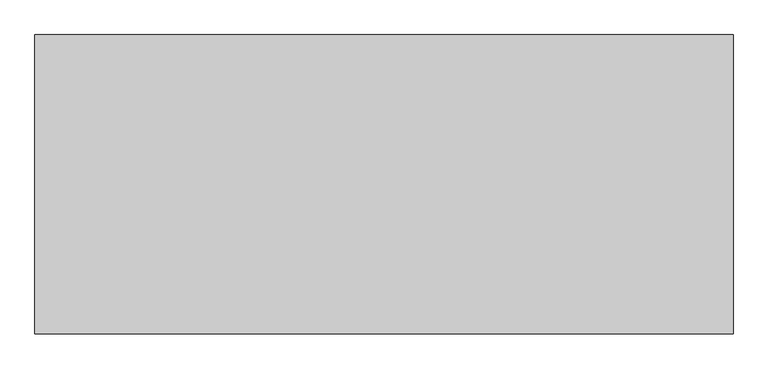
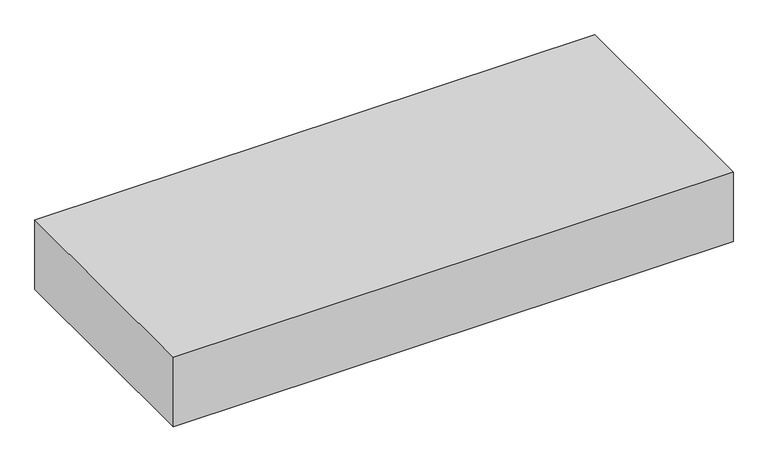
"""IFC4 building model written with IfcOpenShell, lengths in millimetres: proxy geometry, Space Planning Box_hec : Space Planning Box_hec."""

import ifcopenshell
import ifcopenshell.guid

model = None  # the IFC model being written
_history = None  # IfcOwnerHistory: only IFC2X3 demands one
_inside = {}  # id of a spatial element -> (the spatial element, [elements in it])
_under = {}  # id of a project, library or spatial element -> (it, [spatial elements below it])
_declared = {}  # id of a project -> (the project, [libraries it declares])
_typed = {}  # id of a type object -> (the type object, [elements of that type])
_made_of = {}  # id of a material, layer set ... -> (it, [elements and type objects made of it])


def new_model(schema):
    """Start an empty IFC model of exactly this schema.

    Asked for "IFC4X3", IfcOpenShell would pick the latest addendum, in which some entities
    have other attributes; the version numbers below select the first issue.
    IFC2X3 requires an IfcOwnerHistory on every rooted entity: one is made here for all.
    """
    global model, _history
    if schema == "IFC4X3":
        model = ifcopenshell.file(schema_version=(4, 3, 0, 0))
    else:
        model = ifcopenshell.file(schema=schema)
    _inside.clear()
    _under.clear()
    _declared.clear()
    _typed.clear()
    _made_of.clear()
    _history = None
    if model.schema == "IFC2X3":
        org = make("IfcOrganization", Name="unknown")
        user = make(
            "IfcPersonAndOrganization",
            ThePerson=make("IfcPerson", FamilyName="unknown"),
            TheOrganization=org,
        )
        app = make(
            "IfcApplication",
            ApplicationDeveloper=org,
            Version="unknown",
            ApplicationFullName="unknown",
            ApplicationIdentifier="unknown",
        )
        _history = make(
            "IfcOwnerHistory",
            OwningUser=user,
            OwningApplication=app,
            ChangeAction="ADDED",
            CreationDate=0,
        )
    return model


def make(cls, **values):
    """One entity of the class cls with the attributes given. An attribute that is None is left unset."""
    return model.create_entity(
        cls, **{name: value for name, value in values.items() if value is not None}
    )


def rooted(cls, **values):
    """An entity with a GlobalId (a new one), such as an element, a storey or a relation."""
    return make(cls, GlobalId=ifcopenshell.guid.new(), OwnerHistory=_history, **values)


def si_unit(unit_type, name, prefix=None):
    """IfcSIUnit, for example si_unit("LENGTHUNIT", "METRE", prefix="MILLI")."""
    return make("IfcSIUnit", UnitType=unit_type, Prefix=prefix, Name=name)


def assignment(units):
    """IfcUnitAssignment: the units of a project."""
    return None if units is None else make("IfcUnitAssignment", Units=units)


def point(xyz):
    """IfcCartesianPoint."""
    return None if xyz is None else make("IfcCartesianPoint", Coordinates=xyz)


def direction(xyz):
    """IfcDirection."""
    return None if xyz is None else make("IfcDirection", DirectionRatios=xyz)


def frame(location, z_axis=None, x_axis=None):
    """IfcAxis2Placement3D, a coordinate frame: its origin and axes. An axis left out is left unset."""
    return make(
        "IfcAxis2Placement3D",
        Location=point(location),
        Axis=direction(z_axis),
        RefDirection=direction(x_axis),
    )


def origin():
    """The frame at (0, 0, 0) with its axes left unset."""
    return frame((0.0, 0.0, 0.0))


def origin_with_axes():
    """The frame at (0, 0, 0) with the z axis (0, 0, 1) and the x axis (1, 0, 0) written out."""
    return frame((0.0, 0.0, 0.0), z_axis=(0.0, 0.0, 1.0), x_axis=(1.0, 0.0, 0.0))


def place(relative_to, where):
    """IfcLocalPlacement: puts the frame where relative to a parent placement (None: the world)."""
    return make(
        "IfcLocalPlacement", PlacementRelTo=relative_to, RelativePlacement=where
    )


def context(
    kind, dimensions, precision=None, world=None, true_north=None, identifier=None
):
    """IfcGeometricRepresentationContext, for example the 3D "Model" context."""
    return make(
        "IfcGeometricRepresentationContext",
        ContextIdentifier=identifier,
        ContextType=kind,
        CoordinateSpaceDimension=dimensions,
        Precision=precision,
        WorldCoordinateSystem=world,
        TrueNorth=true_north,
    )


def project(units=None, contexts=None):
    """IfcProject with its units and contexts."""
    return rooted(
        "IfcProject",
        Name="project",
        RepresentationContexts=contexts,
        UnitsInContext=assignment(units),
    )


def spatial(cls, under=None, at=None, **own):
    """A site, building, storey or space (cls), placed at a placement, below another one or the project."""
    s = rooted(cls, ObjectPlacement=at, **own)
    if under is not None:
        _under.setdefault(under.id(), (under, []))[1].append(s)
    return s


def polyline(points):
    """IfcPolyline through the points."""
    return make("IfcPolyline", Points=[point(p) for p in points])


def outline(outer, holes=None, kind="AREA"):
    """IfcArbitraryClosedProfileDef: a profile drawn as a closed curve; with holes, ...WithVoids."""
    if holes is None:
        return make("IfcArbitraryClosedProfileDef", ProfileType=kind, OuterCurve=outer)
    return make(
        "IfcArbitraryProfileDefWithVoids",
        ProfileType=kind,
        OuterCurve=outer,
        InnerCurves=holes,
    )


def extrude(swept, where, along, depth):
    """IfcExtrudedAreaSolid: the profile swept, set in the frame where, extruded along a direction by depth."""
    return make(
        "IfcExtrudedAreaSolid",
        SweptArea=swept,
        Position=where,
        ExtrudedDirection=direction(along),
        Depth=depth,
    )


def shape(context_of_items, identifier, shape_type, items):
    """IfcShapeRepresentation: the items that make up one representation, for example the "Body"."""
    return make(
        "IfcShapeRepresentation",
        ContextOfItems=context_of_items,
        RepresentationIdentifier=identifier,
        RepresentationType=shape_type,
        Items=items,
    )


def source(mapping_origin, context_of_items, identifier, shape_type, items):
    """IfcRepresentationMap: a shape defined once, which mapped items show again and again."""
    return make(
        "IfcRepresentationMap",
        MappingOrigin=mapping_origin,
        MappedRepresentation=shape(context_of_items, identifier, shape_type, items),
    )


def transform(
    local_origin,
    x_axis=None,
    y_axis=None,
    z_axis=None,
    scale=None,
    scale2=None,
    scale3=None,
    uniform=True,
):
    """IfcCartesianTransformationOperator3D, or its non-uniform kind. x_axis, y_axis, z_axis: its Axis1, 2, 3."""
    if uniform:
        return make(
            "IfcCartesianTransformationOperator3D",
            Axis1=direction(x_axis),
            Axis2=direction(y_axis),
            LocalOrigin=point(local_origin),
            Scale=scale,
            Axis3=direction(z_axis),
        )
    return make(
        "IfcCartesianTransformationOperator3DnonUniform",
        Axis1=direction(x_axis),
        Axis2=direction(y_axis),
        LocalOrigin=point(local_origin),
        Scale=scale,
        Axis3=direction(z_axis),
        Scale2=scale2,
        Scale3=scale3,
    )


def mapped(mapping_source, mapping_target):
    """IfcMappedItem: shows the shape of a source again, moved by a transform."""
    return make(
        "IfcMappedItem", MappingSource=mapping_source, MappingTarget=mapping_target
    )


def made_of(thing, what):
    """Note that an element or type object is made of a material, layer set ...; save() writes the relation."""
    if what is not None:
        _made_of.setdefault(what.id(), (what, []))[1].append(thing)
    return thing


def element(
    cls,
    number,
    at=None,
    inside=None,
    cuts=None,
    type_object=None,
    material=None,
    context=None,
    identifier="Body",
    shape_type=None,
    held_by="IfcProductDefinitionShape",
    body=None,
    shapes=None,
    **own,
):
    """One element of the class cls, such as IfcWall. Its Tag is "e" and its number.

    at: its placement. inside: the storey or other place that contains it. cuts: it is an
    opening in that element (IfcRelVoidsElement). A single representation is given by context,
    identifier, shape_type and body (its items); several are given by shapes. held_by: the class
    of the entity that holds the representations. save() writes the other relations.
    """
    e = rooted(cls, Tag="e%d" % number, ObjectPlacement=at, **own)
    if body is not None:
        shapes = [shape(context, identifier, shape_type, body)]
    if shapes is not None:
        e.Representation = make(held_by, Representations=shapes)
    if inside is not None:
        _inside.setdefault(inside.id(), (inside, []))[1].append(e)
    if cuts is not None:
        rooted(
            "IfcRelVoidsElement", RelatingBuildingElement=cuts, RelatedOpeningElement=e
        )
    if type_object is not None:
        _typed.setdefault(type_object.id(), (type_object, []))[1].append(e)
    return made_of(e, material)


def aggregate(whole, parts):
    """IfcRelAggregates: a whole, such as a stair, and the parts it consists of."""
    return rooted("IfcRelAggregates", RelatingObject=whole, RelatedObjects=parts)


def save(model, path):
    """Write the relations noted so far, then the file.

    IfcRelAggregates (storeys below a building ...), IfcRelContainedInSpatialStructure (elements
    in a storey), IfcRelDefinesByType, IfcRelAssociatesMaterial and IfcRelDeclares: one each for
    every whole, place, type object, material and project.
    """
    for whole, parts in _under.values():
        aggregate(whole, parts)
    for where, things in _inside.values():
        rooted(
            "IfcRelContainedInSpatialStructure",
            RelatedElements=things,
            RelatingStructure=where,
        )
    for kind, things in _typed.values():
        rooted("IfcRelDefinesByType", RelatedObjects=things, RelatingType=kind)
    for what, things in _made_of.values():
        rooted("IfcRelAssociatesMaterial", RelatedObjects=things, RelatingMaterial=what)
    for by, libraries in _declared.values():
        rooted("IfcRelDeclares", RelatingContext=by, RelatedDefinitions=libraries)
    model.write(path)


def generic_models_3d03af35(model_context):
    return source(origin(), model_context, "Body", "SweptSolid", [
        extrude(outline(polyline([(21000.0, 9000.0), (21000.0, -9000.0), (-21000.0, -9000.0), (-21000.0, 9000.0), (21000.0, 9000.0)])), origin_with_axes(), (0.0, 0.0, 1.0), 5500.0),
    ])


if __name__ == "__main__":
    model = new_model("IFC4")
    model_context = context("Model", 3, world=origin())
    ifc_project = project(units=[si_unit("LENGTHUNIT", "METRE", prefix="MILLI")], contexts=[model_context])
    site = spatial("IfcSite", under=ifc_project)
    building = spatial("IfcBuilding", under=site)
    placement = place(None, origin())
    generic_models_shape = generic_models_3d03af35(model_context)
    element("IfcBuildingElementProxy", 1, Name="Space Planning Box_hec : Space Planning Box_hec", ObjectType="Space Planning Box_hec : Space Planning Box_hec", at=placement, inside=building, context=model_context, shape_type="MappedRepresentation", body=[
        mapped(generic_models_shape, transform((0.0, 0.0, 0.0), x_axis=(1.0, 0.0, 0.0), y_axis=(0.0, 1.0, 0.0), z_axis=(0.0, 0.0, 1.0))),
    ])
    save(model, "model.ifc")

# Revit data of these elements
# Type "Space Planning Box_hec : Space Planning Box_hec"
#   Type Comments = "..."
#   Room Name [instance default] = "?"
#   Interior Finish [instance default] = ""
#   Exterior Finish [instance default] = ""
#   Department [instance default] = ""
#   Assembly Code = "..."
#   ceiling height [instance default] = 0
#   Width [instance default] = 1524 mm
#   Program Area [instance default] = 0.00 m²
#   Length [instance default] = 1524 mm
#   Height [instance default] = 1524 mm
#   Area [instance default] = 2.32258 m²
#   Fill Color [instance default] = Cyan
#   Default Elevation = 0
# Element 1 (IfcBuildingElementProxy, "Space Planning Box_hec : Space Planning Box_hec")
#   Room Name = "Corridor"
#   Exterior Finish = "N/A..N/A,,EW2..N/A..N/A"
#   Department = "AR"
#   Width = 42000 mm
#   Length = 18000 mm
#   Height = 5500 mm
#   Area = 756.00 m²
#   Materials on its faces: "Cyan"
# Materials
#   "Cyan": class "Generic", colour RGB 0 255 255, transparency 0.2, Cost = 0
